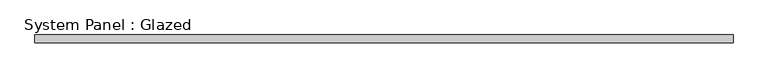
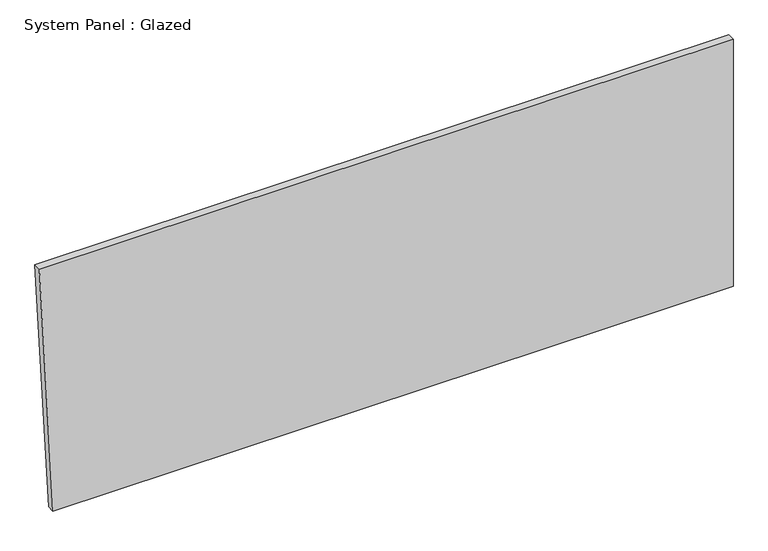
"""IFC4 building model written with IfcOpenShell, lengths in millimetres: plate geometry, System Panel : Glazed."""

from ifc_helpers import new_model, si_unit, frame, origin, place, context, project, spatial, polyline, outline, extrude, source, transform, mapped, element, save


def system_panel_glazed_624ae8a5(model_context):
    return source(origin(), model_context, "Body", "SweptSolid", [
        extrude(outline(polyline([(0.0, -1106.180401), (0.0, 1151.5076076), (866.081558, 1151.5076076), (866.081558, -1151.5076076), (0.0, -1106.180401)])), frame((0.0, -44.45, 0.0), z_axis=(0.0, 1.0, 0.0), x_axis=(0.0, 0.0, 1.0)), (0.0, 0.0, 1.0), 25.4),
    ])


if __name__ == "__main__":
    model = new_model("IFC4")
    model_context = context("Model", 3, world=origin())
    ifc_project = project(units=[si_unit("LENGTHUNIT", "METRE", prefix="MILLI")], contexts=[model_context])
    site = spatial("IfcSite", under=ifc_project)
    building = spatial("IfcBuilding", under=site)
    placement = place(None, origin())
    system_panel_glazed_shape = system_panel_glazed_624ae8a5(model_context)
    element("IfcPlate", 1, ObjectType="System Panel : Glazed", at=placement, inside=building, context=model_context, shape_type="MappedRepresentation", body=[
        mapped(system_panel_glazed_shape, transform((0.0, 0.0, 0.0), x_axis=(1.0, 0.0, 0.0), y_axis=(0.0, 1.0, 0.0), z_axis=(0.0, 0.0, 1.0))),
    ])
    save(model, "model.ifc")

# Revit data of these elements
# Type "System Panel : Glazed"
#   Construction Type Id = "GSP4R"
#   Analytic Construction = "1/8 in Pilkington single glazing"
#   Visual Light Transmittance = 0.9
#   Solar Heat Gain Coefficient = 0.86
#   Heat Transfer Coefficient (U) = 1.18115 BTU/(h·ft²·°F)
#   Define Thermal Properties by = 1
# Element 1 (IfcPlate, "System Panel : Glazed")
#   Materials on its faces: "Glass"
# Materials
#   "Glass": class "Glass", colour RGB 0 128 192, transparency 0.75, Description = "Soda Lime Glass", Cost = 0
